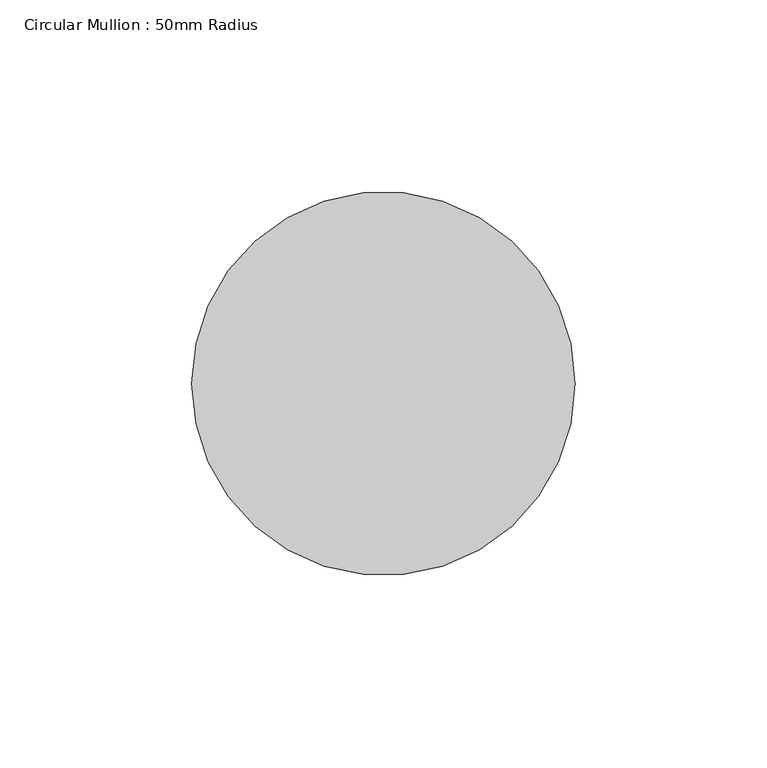
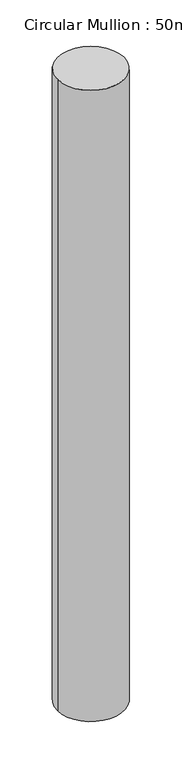
"""IFC4 building model written with IfcOpenShell, lengths in millimetres: member geometry, Circular Mullion : 50mm Radius."""

from ifc_helpers import new_model, si_unit, point, frame, origin, origin_2d, place, context, project, spatial, circle_curve, trimmed, segment, composite_curve, outline, extrude, source, transform, mapped, element, save


def circular_mullion_50mm_radius_cd73be27(model_context):
    return source(origin(), model_context, "Body", "SweptSolid", [
        extrude(outline(composite_curve([segment(trimmed(circle_curve(origin_2d(), 50.0), [point((50.0, 0.0))], [point((-50.0, 0.0))], False, "CARTESIAN"), True, "CONTINUOUS"), segment(trimmed(circle_curve(origin_2d(), 50.0), [point((-50.0, 0.0))], [point((50.0, 0.0))], False, "CARTESIAN"), True, "CONTINUOUS")], self_intersect=False)), frame((0.0, 0.0, -1003.9384833), z_axis=(0.0, 0.0, 1.0), x_axis=(1.0, 0.0, 0.0)), (0.0, 0.0, 1.0), 1003.9384833),
    ])


if __name__ == "__main__":
    model = new_model("IFC4")
    model_context = context("Model", 3, world=origin())
    ifc_project = project(units=[si_unit("LENGTHUNIT", "METRE", prefix="MILLI")], contexts=[model_context])
    site = spatial("IfcSite", under=ifc_project)
    building = spatial("IfcBuilding", under=site)
    placement = place(None, origin())
    circular_mullion_50mm_radius_shape = circular_mullion_50mm_radius_cd73be27(model_context)
    element("IfcMember", 1, ObjectType="Circular Mullion : 50mm Radius", at=placement, inside=building, context=model_context, shape_type="MappedRepresentation", body=[
        mapped(circular_mullion_50mm_radius_shape, transform((0.0, 0.0, 0.0), x_axis=(1.0, 0.0, 0.0), y_axis=(0.0, 1.0, 0.0), z_axis=(0.0, 0.0, 1.0))),
    ])
    save(model, "model.ifc")

# Revit data of these elements
# Type "Circular Mullion : 50mm Radius"
#   built-in parameter 1007350 = 0.164042 (stored number, unit not read)
# Element 1 (IfcMember, "Circular Mullion : 50mm Radius")
#   Materials on its faces: "Aluminium"
# Materials
#   "Aluminium": class "Metal", colour RGB 247 247 247, transparency 0, Description = "Aluminium 6061", Cost = 0
